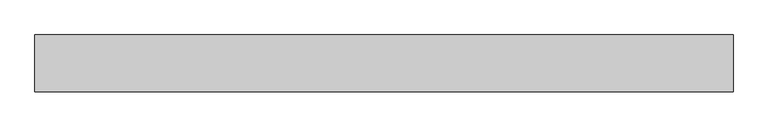
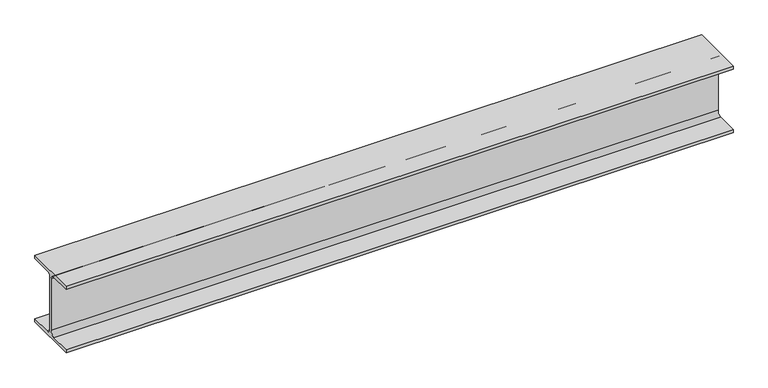
"""IFC4 building model written with IfcOpenShell, lengths in millimetres: beam geometry, 0912_Steel Framing_H-KSD3502 : H_SB_ASB_H-194x150x6x9."""

from ifc_helpers import new_model, si_unit, point, frame, frame_2d, origin, place, context, project, spatial, polyline, circle_curve, trimmed, segment, composite_curve, outline, extrude, source, transform, mapped, element, save


def beam_61d1b7df(model_context):
    return source(origin(), model_context, "Body", "SweptSolid", [
        extrude(outline(composite_curve([segment(polyline([(-75.0, -88.0), (-16.0, -88.0)]), True, "CONTINUOUS"), segment(trimmed(circle_curve(frame_2d((-16.0, -75.0)), 13.0), [point((-16.0, -88.0))], [point((-3.0, -75.0))], True, "CARTESIAN"), True, "CONTINUOUS"), segment(polyline([(-3.0, -75.0), (-3.0, 75.0)]), True, "CONTINUOUS"), segment(trimmed(circle_curve(frame_2d((-16.0, 75.0)), 13.0), [point((-3.0, 75.0))], [point((-16.0, 88.0))], True, "CARTESIAN"), True, "CONTINUOUS"), segment(polyline([(-16.0, 88.0), (-75.0, 88.0), (-75.0, 97.0), (75.0, 97.0), (75.0, 88.0), (16.0, 88.0)]), True, "CONTINUOUS"), segment(trimmed(circle_curve(frame_2d((16.0, 75.0)), 13.0), [point((16.0, 88.0))], [point((3.0, 75.0))], True, "CARTESIAN"), True, "CONTINUOUS"), segment(polyline([(3.0, 75.0), (3.0, -75.0)]), True, "CONTINUOUS"), segment(trimmed(circle_curve(frame_2d((16.0, -75.0)), 13.0), [point((3.0, -75.0))], [point((16.0, -88.0))], True, "CARTESIAN"), True, "CONTINUOUS"), segment(polyline([(16.0, -88.0), (75.0, -88.0), (75.0, -97.0), (-75.0, -97.0), (-75.0, -88.0)]), True, "CONTINUOUS")], self_intersect=False)), frame((-851.3274068, 0.0, 0.0), z_axis=(1.0, 0.0, 0.0), x_axis=(0.0, 1.0, 0.0)), (0.0, 0.0, 1.0), 1839.6820153),
    ])


if __name__ == "__main__":
    model = new_model("IFC4")
    model_context = context("Model", 3, world=origin())
    ifc_project = project(units=[si_unit("LENGTHUNIT", "METRE", prefix="MILLI")], contexts=[model_context])
    site = spatial("IfcSite", under=ifc_project)
    building = spatial("IfcBuilding", under=site)
    placement = place(None, origin())
    beam_shape = beam_61d1b7df(model_context)
    element("IfcBeam", 1, ObjectType="0912_Steel Framing_H-KSD3502 : H_SB_ASB_H-194x150x6x9", at=placement, inside=building, context=model_context, shape_type="MappedRepresentation", body=[
        mapped(beam_shape, transform((0.0, 0.0, 0.0), x_axis=(1.0, 0.0, 0.0), y_axis=(0.0, 1.0, 0.0), z_axis=(0.0, 0.0, 1.0))),
    ])
    save(model, "model.ifc")

# Revit data of these elements
# Type "0912_Steel Framing_H-KSD3502 : H_SB_ASB_H-194x150x6x9"
#   H_WM Code_1 = "S01AA002-00001 | Main Steel Structure Fabrication Work | Shelter/Building | Medium Steel - Standard (90KG/M>Weight≥30KG/M) | Material: (   )"
#   H_WM Code_2 = "S03AA028-00001 | Main Steel Structure Erection Work | Shelter/Building | Medium Steel (90KG/M>Weight≥30KG/M) | Material: (   )"
#   H_WM Code_3 = "S01AA010-00001 | Main Steel Structure Fabrication Work | Shelter/Building | Steel Painting/Coating | for Non-Fireproofed Steel Surface, Surface Preparation, Primer, Second & Final Coat | Material: (   )"
#   H_Q'ty Cal Type Tag = "SB-Q2"
#   Width = 15.0 cm
#   Web Thickness = 0.6 cm
#   Web Fillet = 1.3 cm
#   Warping Constant = 43316.0 cm⁶
#   W = 0
#   Torsional Moment of Inertia = 8.622 cm⁴
#   Section Area = 39.01 cm²
#   Plastic Modulus weak axis = 104.0 cm³
#   Plastic Modulus strong axis = 309.0 cm³
#   Perimeter = 0.95 m²/m
#   Nominal Weight = 30.60 kgf/m
#   Moment of Inertia weak axis = 507.00 cm⁴
#   Moment of Inertia strong axis = 2690.00 cm⁴
#   Height = 19.4 cm
#   Flange Thickness = 0.9 cm
#   Elastic Modulus weak axis = 67.6 cm³
#   Elastic Modulus strong axis = 277.0 cm³
#   Centroid Vertical = 9.7 cm
#   Centroid Horizontal = 7.5 cm
#   Ix = 26900000
#   Length [instance default] = 1.5240 m
#   Zx = 309000
#   b = 0.1500 m
#   h = 0.1940 m
#   r = 0.0130 m
#   s = 0.0060 m
#   t = 0.0090 m
#   A = 0.003901 m²
#   Structural Material [instance default] = Steel, 45-345
#   Assembly Code = ""
# Element 1 (IfcBeam, "0912_Steel Framing_H-KSD3502 : H_SB_ASB_H-194x150x6x9")
#   Structural Material = none
# Materials
#   "Steel, 45-345": class "Metal", colour RGB 189 187 185, transparency 0, Description = "Steel 345 MPa", Cost = 0
